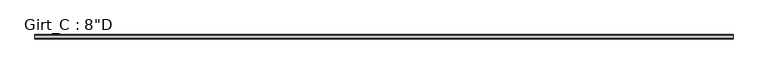
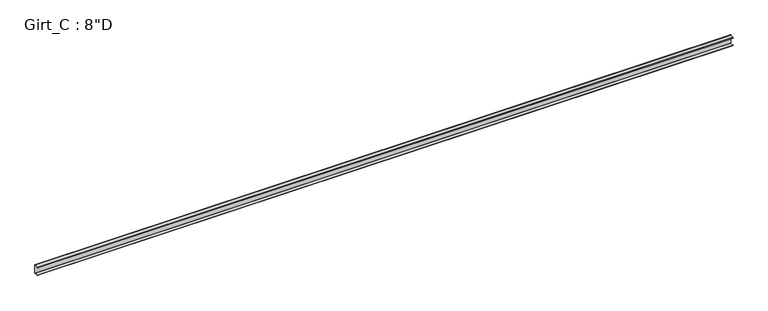
"""IFC4 building model written with IfcOpenShell, lengths in millimetres: beam geometry."""

from ifc_helpers import new_model, si_unit, point, frame, frame_2d, origin, place, context, project, spatial, polyline, circle_curve, trimmed, segment, composite_curve, outline, extrude, source, transform, mapped, element, save


def beam_cf5de932(model_context):
    return source(origin(), model_context, "Body", "SweptSolid", [
        extrude(outline(composite_curve([segment(polyline([(-87.5109375, 101.6), (-3.3734375, 101.6)]), True, "CONTINUOUS"), segment(trimmed(circle_curve(frame_2d((-3.3734375, 96.8375)), 4.7625), [point((-3.3734375, 101.6))], [point((1.3890625, 96.8375))], False, "CARTESIAN"), True, "CONTINUOUS"), segment(polyline([(1.3890625, 96.8375), (1.3890625, -96.8375)]), True, "CONTINUOUS"), segment(trimmed(circle_curve(frame_2d((-3.3734375, -96.8375)), 4.7625), [point((1.3890625, -96.8375))], [point((-3.3734375, -101.6))], False, "CARTESIAN"), True, "CONTINUOUS"), segment(polyline([(-3.3734375, -101.6), (-87.5109375, -101.6), (-99.7792647, -86.979177), (-97.6510975, -85.1934327), (-86.2154765, -98.821875), (-3.2694106, -98.821875)]), True, "CONTINUOUS"), segment(trimmed(circle_curve(frame_2d((-3.3748024, -96.8389339)), 1.9857399), [point((-3.2694106, -98.821875))], [point((-1.3890625, -96.8389339))], True, "CARTESIAN"), True, "CONTINUOUS"), segment(polyline([(-1.3890625, -96.8389339), (-1.3890625, 96.8381931)]), True, "CONTINUOUS"), segment(trimmed(circle_curve(frame_2d((-3.3741066, 96.8381931)), 1.9850441), [point((-1.3890625, 96.8381931))], [point((-3.3005807, 98.821875))], True, "CARTESIAN"), True, "CONTINUOUS"), segment(polyline([(-3.3005807, 98.821875), (-86.2154765, 98.821875), (-97.6278742, 85.221109), (-99.7560415, 87.0068534), (-87.5109375, 101.6)]), True, "CONTINUOUS")], self_intersect=False)), frame((-7955.1935059, 0.0, 0.0), z_axis=(1.0, 0.0, 0.0), x_axis=(0.0, 1.0, 0.0)), (0.0, 0.0, 1.0), 15846.1237787),
    ])


if __name__ == "__main__":
    model = new_model("IFC4")
    model_context = context("Model", 3, world=origin())
    ifc_project = project(units=[si_unit("LENGTHUNIT", "METRE", prefix="MILLI")], contexts=[model_context])
    site = spatial("IfcSite", under=ifc_project)
    building = spatial("IfcBuilding", under=site)
    placement = place(None, origin())
    beam_shape = beam_cf5de932(model_context)
    element("IfcBeam", 1, ObjectType="Girt_C : 8\"D", at=placement, inside=building, context=model_context, shape_type="MappedRepresentation", body=[
        mapped(beam_shape, transform((0.0, 0.0, 0.0), x_axis=(1.0, 0.0, 0.0), y_axis=(0.0, 1.0, 0.0), z_axis=(0.0, 0.0, 1.0))),
    ])
    save(model, "model.ifc")

# Revit data of these elements
# Type "Girt_C : 8\"D"
#   half leg = 0' - 1 3/4"
#   Web_Thickness = 0' - 0 7/64"
#   Length [instance default] = 10' - 0"
#   Leg_1 = 0' - 3 1/2"
#   Height = 0' - 8"
#   Structural Material [instance default] = none
# Element 1 (IfcBeam, "Girt_C : 8\"D")
#   Structural Material = GALVANIZED 'CEE' SECTION (8.0x3.5C - SEE STRUCT. DWGS)
#   Materials on its faces: "GALVANIZED 'CEE' SECTION (8.0x3.5C - SEE STRUCT. DWGS)"
# Materials
#   "GALVANIZED 'CEE' SECTION (8.0x3.5C - SEE STRUCT. DWGS)": class "Metal", colour RGB 137 146 153, transparency 0, Description = "Steel, mill finish", Cost = 0
